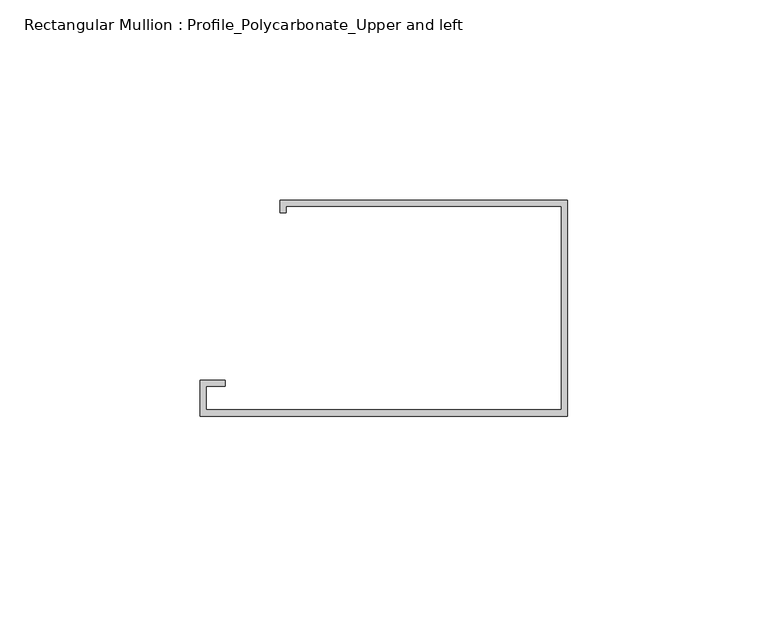
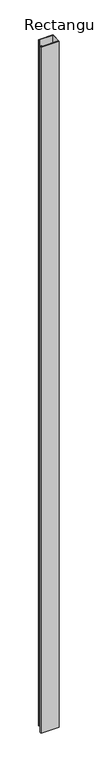
"""IFC4 building model written with IfcOpenShell, lengths in millimetres: member geometry, Rectangular Mullion : Profile_Polycarbonate_Upper and left."""

from ifc_helpers import new_model, si_unit, frame, origin, place, context, project, spatial, polyline, outline, extrude, source, transform, mapped, element, save


def rectangular_mullion_profile_polycarbonate_upper_and_left_d43e69b3(model_context):
    return source(origin(), model_context, "Body", "SweptSolid", [
        extrude(outline(polyline([(0.0, -28.984575), (-91.9988, -28.984575), (-91.9988, -19.992975), (-85.6488, -19.992975), (-85.6488, -21.580475), (-90.4113, -21.580475), (-90.4113, -27.397075), (-1.5875, -27.397075), (-1.5875, 23.428325), (-70.3961, 23.428325), (-70.3961, 21.840825), (-71.9836, 21.840825), (-71.9836, 25.015825), (0.0, 25.015825), (0.0, -28.984575)])), frame((0.0, 0.0, -3657.6), z_axis=(0.0, 0.0, 1.0), x_axis=(1.0, 0.0, 0.0)), (0.0, 0.0, 1.0), 3657.6),
    ])


if __name__ == "__main__":
    model = new_model("IFC4")
    model_context = context("Model", 3, world=origin())
    ifc_project = project(units=[si_unit("LENGTHUNIT", "METRE", prefix="MILLI")], contexts=[model_context])
    site = spatial("IfcSite", under=ifc_project)
    building = spatial("IfcBuilding", under=site)
    placement = place(None, origin())
    rectangular_mullion_profile_polycarbonate_upper_and_left_shape = rectangular_mullion_profile_polycarbonate_upper_and_left_d43e69b3(model_context)
    element("IfcMember", 1, ObjectType="Rectangular Mullion : Profile_Polycarbonate_Upper and left", at=placement, inside=building, context=model_context, shape_type="MappedRepresentation", body=[
        mapped(rectangular_mullion_profile_polycarbonate_upper_and_left_shape, transform((0.0, 0.0, 0.0), x_axis=(1.0, 0.0, 0.0), y_axis=(0.0, 1.0, 0.0), z_axis=(0.0, 0.0, 1.0))),
    ])
    save(model, "model.ifc")

# Revit data of these elements
# Type "Rectangular Mullion : Profile_Polycarbonate_Upper and left"
#   built-in parameter 1007322 = 0.177167 (stored number, unit not read)
#   built-in parameter 1007321 = 0.00520833 (stored number, unit not read)
#   built-in parameter 1007320 = 0 (stored number, unit not read)
